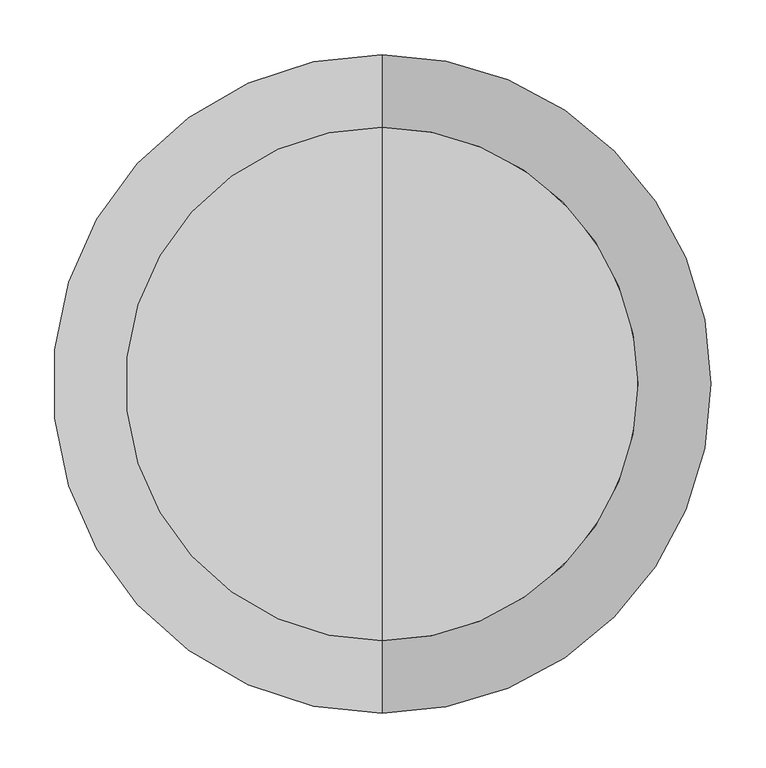
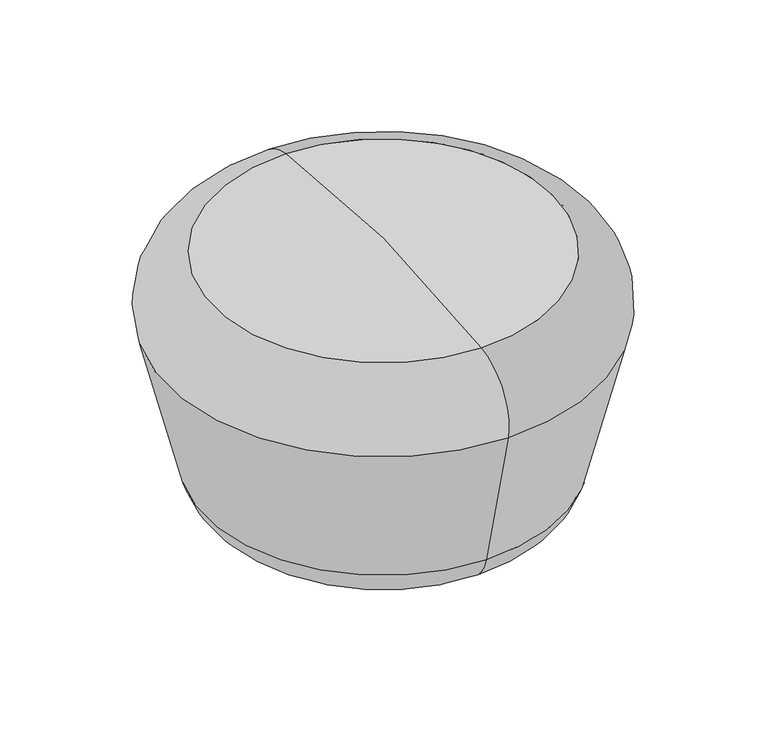
"""IFC4 building model written with IfcOpenShell, lengths in millimetres: furniture geometry, puf_13251 : puff."""

from ifc_helpers import new_model, si_unit, point, frame, origin, place, context, project, spatial, polyline, circle_curve, ellipse_curve, trimmed, source, transform, mapped, element, save
from ifc_brep_helpers import plane_surface, revolved_surface, advanced_brep


def furniture_ba43957c(model_context):
    return source(origin(), model_context, "Body", "AdvancedBrep", [
        advanced_brep(
        [(0.0, -178.4134503, 0.0), (0.0, 178.4134503, 0.0), (0.0, 0.0, 0.0), (0.0, -246.3234253, 53.0225062), (0.0, 246.3234253, 53.0225062), (0.0, -298.9734658, 263.6226683), (0.0, 298.9734658, 263.6226683), (0.0, -234.791561, 356.320588), (0.0, 234.791561, 356.320588), (0.0, 0.0, 375.0541427)],
        [
            (0, 1, circle_curve(frame((0.0, 0.0, 0.0), z_axis=(0.0, 0.0, -1.0), x_axis=(0.0, 1.0, 0.0)), 178.4134503)),
            (1, 2),
            (2, 0),
            (1, 0, circle_curve(frame((0.0, 0.0, 0.0), z_axis=(0.0, 0.0, -1.0), x_axis=(0.0, 1.0, 0.0)), 178.4134503)),
            (3, 4, circle_curve(frame((0.0, 0.0, 53.0225062), z_axis=(0.0, 0.0, -1.0), x_axis=(0.0, 1.0, 0.0)), 246.3234253)),
            (4, 1, circle_curve(frame((0.0, 178.4134503, 70.0), z_axis=(-1.0, 0.0, 0.0), x_axis=(0.0, 1.0, 0.0)), 70.0)),
            (0, 3, circle_curve(frame((0.0, -178.4134503, 70.0), z_axis=(-1.0, 0.0, 0.0), x_axis=(0.0, -1.0, 0.0)), 70.0)),
            (4, 3, circle_curve(frame((0.0, 0.0, 53.0225062), z_axis=(0.0, 0.0, -1.0), x_axis=(0.0, 1.0, 0.0)), 246.3234253)),
            (5, 6, circle_curve(frame((0.0, 0.0, 263.6226683), z_axis=(0.0, 0.0, -1.0), x_axis=(0.0, 1.0, 0.0)), 298.9734658)),
            (6, 4),
            (3, 5),
            (6, 5, circle_curve(frame((0.0, 0.0, 263.6226683), z_axis=(0.0, 0.0, -1.0), x_axis=(0.0, 1.0, 0.0)), 298.9734658)),
            (7, 8, circle_curve(frame((0.0, 0.0, 356.320588), z_axis=(0.0, 0.0, -1.0), x_axis=(0.0, 1.0, 0.0)), 234.791561)),
            (8, 6, circle_curve(frame((0.0, 226.2127783, 281.8128402), z_axis=(-1.0, 0.0, 0.0), x_axis=(0.0, 1.0, 0.0)), 75.0)),
            (5, 7, circle_curve(frame((0.0, -226.2127783, 281.8128402), z_axis=(-1.0, 0.0, 0.0), x_axis=(0.0, -1.0, 0.0)), 75.0)),
            (8, 7, circle_curve(frame((0.0, 0.0, 356.320588), z_axis=(0.0, 0.0, -1.0), x_axis=(0.0, 1.0, 0.0)), 234.791561)),
            (9, 8, circle_curve(frame((0.0, -150.0, -2985.6398993), z_axis=(-1.0, 0.0, 0.0), x_axis=(0.0, 1.0, 0.0)), 3364.0398993)),
            (7, 9, circle_curve(frame((0.0, 150.0, -2985.6398993), z_axis=(-1.0, 0.0, 0.0), x_axis=(0.0, -1.0, 0.0)), 3364.0398993)),
        ],
        [
            plane_surface(frame((0.0, 0.0, 0.0), z_axis=(0.0, 0.0, -1.0), x_axis=(0.0, 1.0, 0.0))),
            revolved_surface(trimmed(ellipse_curve(frame((0.0, 178.4134503, 70.0), z_axis=(1.0, 0.0, 0.0), x_axis=(0.0, 1.0, 0.0)), 70.0, 70.0), [point((0.0, 178.4134503, 0.0))], [point((0.0, 246.3234253, 53.0225062))], True, "CARTESIAN"), (0.0, 0.0, 320.0204891), (0.0, 0.0, 1.0)),
            revolved_surface(polyline([(0.0, 246.3234253, 53.0225062), (0.0, 298.9734658, 263.6226683)]), (0.0, 0.0, 320.0204891), (0.0, 0.0, 1.0)),
            revolved_surface(trimmed(ellipse_curve(frame((0.0, 226.2127783, 281.8128402), z_axis=(1.0, 0.0, 0.0), x_axis=(0.0, 1.0, 0.0)), 75.0, 75.0), [point((0.0, 298.9734658, 263.6226683))], [point((0.0, 234.791561, 356.320588))], True, "CARTESIAN"), (0.0, 0.0, 320.0204891), (0.0, 0.0, 1.0)),
            revolved_surface(trimmed(ellipse_curve(frame((0.0, -150.0, -2985.6398993), z_axis=(1.0, 0.0, 0.0), x_axis=(0.0, 1.0, 0.0)), 3364.0398993, 3364.0398993), [point((0.0, 234.791561, 356.320588))], [point((0.0, 0.0, 375.0541427))], True, "CARTESIAN"), (0.0, 0.0, 320.0204891), (0.0, 0.0, 1.0)),
        ],
        [
            (0, [[1, 2, 3]]),
            (0, [[4, -3, -2]]),
            (1, [[5, 6, -1, 7]]),
            (1, [[8, -7, -4, -6]]),
            (2, [[9, 10, -5, 11]]),
            (2, [[12, -11, -8, -10]]),
            (3, [[13, 14, -9, 15]]),
            (3, [[16, -15, -12, -14]]),
            (4, [[17, -13, 18]]),
            (4, [[-18, -16, -17]]),
        ],
    ),
    ])


if __name__ == "__main__":
    model = new_model("IFC4")
    model_context = context("Model", 3, world=origin())
    ifc_project = project(units=[si_unit("LENGTHUNIT", "METRE", prefix="MILLI")], contexts=[model_context])
    site = spatial("IfcSite", under=ifc_project)
    building = spatial("IfcBuilding", under=site)
    placement = place(None, origin())
    furniture_shape = furniture_ba43957c(model_context)
    element("IfcFurniture", 1, ObjectType="puf_13251 : puff", at=placement, inside=building, context=model_context, shape_type="MappedRepresentation", body=[
        mapped(furniture_shape, transform((0.0, 0.0, 0.0), x_axis=(1.0, 0.0, 0.0), y_axis=(0.0, 1.0, 0.0), z_axis=(0.0, 0.0, 1.0))),
    ])
    save(model, "model.ifc")

# Revit data of these elements
# Type "puf_13251 : puff"
#   free02 fabric = free02 fabric
#   Default Elevation = 0
#   Assembly Code = ""
# Element 1 (IfcFurniture, "puf_13251 : puff")
#   Materials on its faces: "free02 fabric"
# Materials
#   "free02 fabric": class "Fabric", colour RGB 56 46 37, transparency 0, Cost = 0
